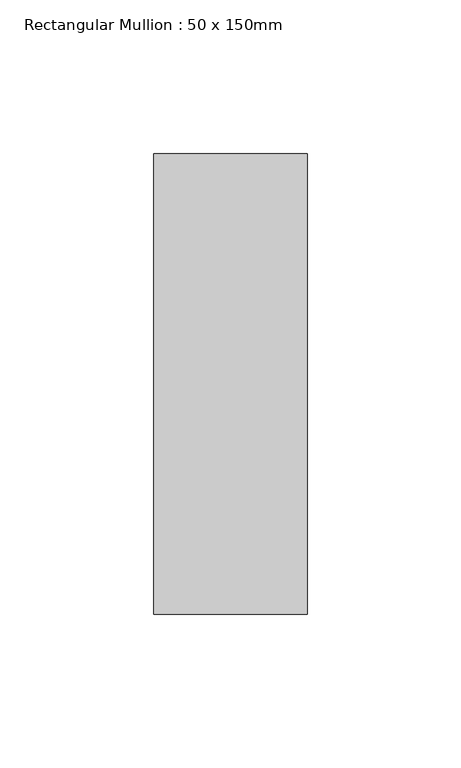
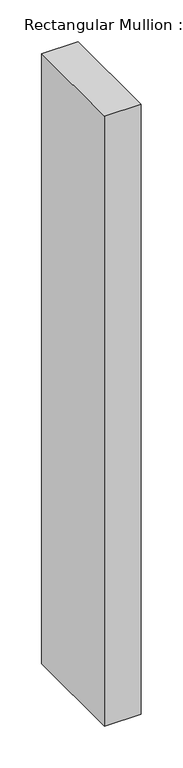
"""IFC4 building model written with IfcOpenShell, lengths in millimetres: member geometry, Rectangular Mullion : 50 x 150mm."""

from ifc_helpers import new_model, si_unit, frame, origin, place, context, project, spatial, polyline, outline, extrude, source, transform, mapped, element, save


def rectangular_mullion_50_x_150mm_6e645c27(model_context):
    return source(origin(), model_context, "Body", "SweptSolid", [
        extrude(outline(polyline([(25.0, 75.0), (25.0, -75.0), (-25.0, -75.0), (-25.0, 75.0), (25.0, 75.0)])), frame((0.0, 0.0, -887.5), z_axis=(0.0, 0.0, 1.0), x_axis=(1.0, 0.0, 0.0)), (0.0, 0.0, 1.0), 887.5),
    ])


if __name__ == "__main__":
    model = new_model("IFC4")
    model_context = context("Model", 3, world=origin())
    ifc_project = project(units=[si_unit("LENGTHUNIT", "METRE", prefix="MILLI")], contexts=[model_context])
    site = spatial("IfcSite", under=ifc_project)
    building = spatial("IfcBuilding", under=site)
    placement = place(None, origin())
    rectangular_mullion_50_x_150mm_shape = rectangular_mullion_50_x_150mm_6e645c27(model_context)
    element("IfcMember", 1, ObjectType="Rectangular Mullion : 50 x 150mm", at=placement, inside=building, context=model_context, shape_type="MappedRepresentation", body=[
        mapped(rectangular_mullion_50_x_150mm_shape, transform((0.0, 0.0, 0.0), x_axis=(1.0, 0.0, 0.0), y_axis=(0.0, 1.0, 0.0), z_axis=(0.0, 0.0, 1.0))),
    ])
    save(model, "model.ifc")

# Revit data of these elements
# Type "Rectangular Mullion : 50 x 150mm"
#   built-in parameter 1007304 = 0.492126 (stored number, unit not read)
#   built-in parameter 1007301 = 0.082021 (stored number, unit not read)
#   built-in parameter 1007300 = 0.082021 (stored number, unit not read)
# Element 1 (IfcMember, "Rectangular Mullion : 50 x 150mm")
#   Materials on its faces: "Aluminium"
# Materials
#   "Aluminium": class "Metal", colour RGB 247 247 247, transparency 0, Description = "Aluminium 6061", Cost = 0
